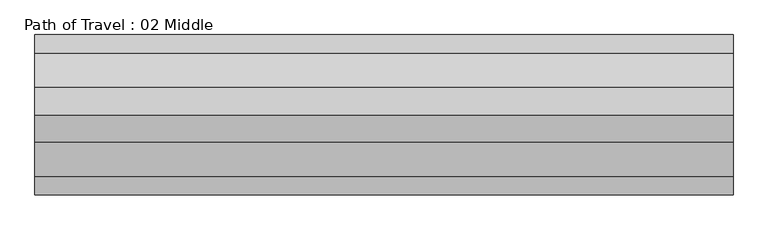
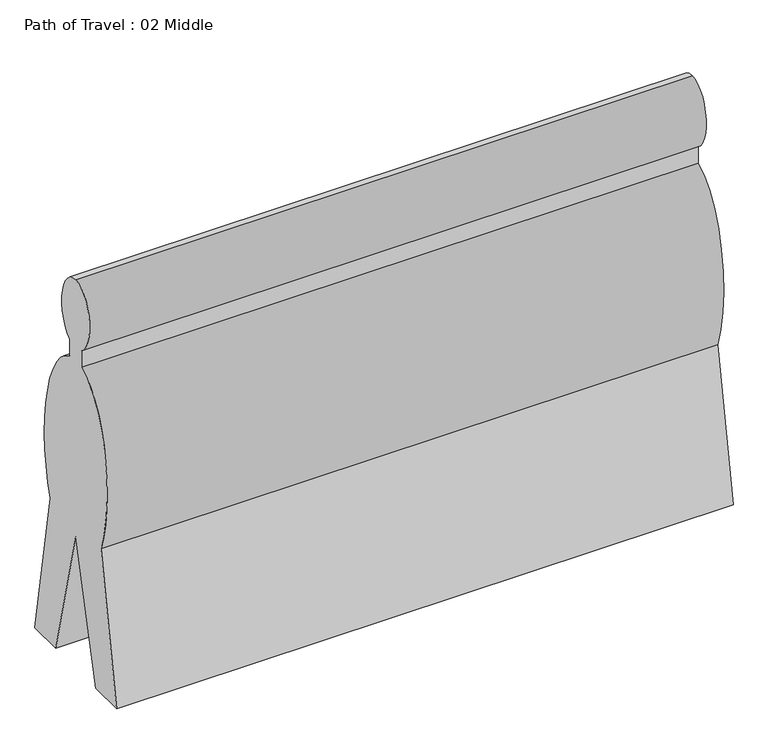
"""IFC4 building model written with IfcOpenShell, lengths in millimetres: proxy geometry, Path of Travel : 02 Middle."""

from ifc_helpers import new_model, si_unit, point, frame, origin, place, context, project, spatial, ellipse_curve, trimmed, source, transform, mapped, element, save
from ifc_brep_helpers import plane_surface, extruded_surface, advanced_brep


def path_of_travel_02_middle_fab60197(model_context):
    return source(origin(), model_context, "Body", "AdvancedBrep", [
        advanced_brep(
        [(227.5554837, 0.0, 1727.2), (227.5554837, 42.9018657, 1436.6534209), (227.5554837, 42.9018657, 1363.4763406), (227.5554837, 184.1186263, 643.4144547), (227.5554837, 297.5699544, 0.0), (227.5554837, 145.6574193, 0.0), (227.5554837, 0.0, 584.2), (227.5554837, -145.6574193, 0.0), (227.5554837, -297.5699544, 0.0), (227.5554837, -184.1186263, 643.4144547), (227.5554837, -42.9018657, 1363.4763406), (227.5554837, -42.9018657, 1436.6534209), (2818.3554837, 0.0, 1727.2), (2818.3554837, -42.9018657, 1436.6534209), (2818.3554837, -42.9018657, 1363.4763406), (2818.3554837, -184.1186263, 643.4144547), (2818.3554837, -297.5699544, 0.0), (2818.3554837, -145.6574193, 0.0), (2818.3554837, 0.0, 584.2), (2818.3554837, 145.6574193, 0.0), (2818.3554837, 297.5699544, 0.0), (2818.3554837, 184.1186263, 643.4144547), (2818.3554837, 42.9018657, 1363.4763406), (2818.3554837, 42.9018657, 1436.6534209)],
        [
            (0, 1, ellipse_curve(frame((227.5554837, 0.0, 1574.8), z_axis=(-1.0, 0.0, 0.0), x_axis=(0.0, 0.0, 1.0)), 152.4, 101.6)),
            (1, 2),
            (2, 3, ellipse_curve(frame((227.5554837, 0.0, 914.4), z_axis=(-1.0, 0.0, 0.0), x_axis=(0.0, 0.0, -1.0)), 457.2, 228.6)),
            (3, 4),
            (4, 5),
            (5, 6),
            (6, 7),
            (7, 8),
            (8, 9),
            (9, 10, ellipse_curve(frame((227.5554837, 0.0, 914.4), z_axis=(-1.0, 0.0, 0.0), x_axis=(0.0, 0.0, -1.0)), 457.2, 228.6)),
            (10, 11),
            (11, 0, ellipse_curve(frame((227.5554837, 0.0, 1574.8), z_axis=(-1.0, 0.0, 0.0), x_axis=(0.0, 0.0, 1.0)), 152.4, 101.6)),
            (12, 13, ellipse_curve(frame((2818.3554837, 0.0, 1574.8), z_axis=(1.0, 0.0, 0.0), x_axis=(0.0, 0.0, 1.0)), 152.4, 101.6)),
            (13, 14),
            (14, 15, ellipse_curve(frame((2818.3554837, 0.0, 914.4), z_axis=(1.0, 0.0, 0.0), x_axis=(0.0, 0.0, -1.0)), 457.2, 228.6)),
            (15, 16),
            (16, 17),
            (17, 18),
            (18, 19),
            (19, 20),
            (20, 21),
            (21, 22, ellipse_curve(frame((2818.3554837, 0.0, 914.4), z_axis=(1.0, 0.0, 0.0), x_axis=(0.0, 0.0, -1.0)), 457.2, 228.6)),
            (22, 23),
            (23, 12, ellipse_curve(frame((2818.3554837, 0.0, 1574.8), z_axis=(1.0, 0.0, 0.0), x_axis=(0.0, 0.0, 1.0)), 152.4, 101.6)),
            (0, 12),
            (23, 1),
            (22, 2),
            (21, 3),
            (20, 4),
            (19, 5),
            (18, 6),
            (17, 7),
            (16, 8),
            (15, 9),
            (14, 10),
            (13, 11),
        ],
        [
            plane_surface(frame((227.5554837, 0.0, 0.0), z_axis=(-1.0, 0.0, 0.0), x_axis=(0.0, 0.0, 1.0))),
            plane_surface(frame((2818.3554837, 0.0, 0.0), z_axis=(1.0, 0.0, 0.0), x_axis=(0.0, 0.0, 1.0))),
            extruded_surface(trimmed(ellipse_curve(frame((2818.3554837, 0.0, 1574.8), z_axis=(-1.0, 0.0, 0.0), x_axis=(0.0, 0.0, 1.0)), 152.4, 101.6), [point((2818.3554837, 0.0, 1727.2))], [point((2818.3554837, 42.9018657, 1436.6534209))], True, "CARTESIAN"), (-2590.8, 0.0, 0.0), 2590.8),
            plane_surface(frame((227.5554837, 42.9018657, 1436.6534209), z_axis=(0.0, 1.0, 0.0), x_axis=(1.0, 0.0, 0.0))),
            extruded_surface(trimmed(ellipse_curve(frame((2818.3554837, 0.0, 914.4), z_axis=(-1.0, 0.0, 0.0), x_axis=(0.0, 0.0, -1.0)), 457.2, 228.6), [point((2818.3554837, 42.9018657, 1363.4763406))], [point((2818.3554837, 184.1186263, 643.4144547))], True, "CARTESIAN"), (-2590.8, 0.0, 0.0), 2590.8),
            plane_surface(frame((227.5554837, 184.1186263, 643.4144547), z_axis=(0.0, 0.9848077530122078, 0.17364817766693205), x_axis=(1.0, 0.0, 0.0))),
            plane_surface(frame((227.5554837, 297.5699544, 0.0), z_axis=(0.0, 0.0, -1.0), x_axis=(1.0, 0.0, 0.0))),
            plane_surface(frame((227.5554837, 145.6574193, 0.0), z_axis=(0.0, -0.9702957262760199, -0.2419218955995739), x_axis=(1.0, 0.0, 0.0))),
            plane_surface(frame((227.5554837, 0.0, 584.2), z_axis=(0.0, 0.9702957262759961, -0.24192189559966923), x_axis=(1.0, 0.0, 0.0))),
            plane_surface(frame((227.5554837, -145.6574193, 0.0), z_axis=(0.0, 0.0, -1.0), x_axis=(1.0, 0.0, 0.0))),
            plane_surface(frame((227.5554837, -297.5699544, 0.0), z_axis=(0.0, -0.984807753012208, 0.17364817766693066), x_axis=(1.0, 0.0, 0.0))),
            extruded_surface(trimmed(ellipse_curve(frame((2818.3554837, 0.0, 914.4), z_axis=(-1.0, 0.0, 0.0), x_axis=(0.0, 0.0, -1.0)), 457.2, 228.6), [point((2818.3554837, -184.1186263, 643.4144547))], [point((2818.3554837, -42.9018657, 1363.4763406))], True, "CARTESIAN"), (-2590.8, 0.0, 0.0), 2590.8),
            plane_surface(frame((227.5554837, -42.9018657, 1363.4763406), z_axis=(0.0, -1.0, 0.0), x_axis=(1.0, 0.0, 0.0))),
            extruded_surface(trimmed(ellipse_curve(frame((2818.3554837, 0.0, 1574.8), z_axis=(-1.0, 0.0, 0.0), x_axis=(0.0, 0.0, 1.0)), 152.4, 101.6), [point((2818.3554837, -42.9018657, 1436.6534209))], [point((2818.3554837, 0.0, 1727.2))], True, "CARTESIAN"), (-2590.8, 0.0, 0.0), 2590.8),
        ],
        [
            (0, [[1, 2, 3, 4, 5, 6, 7, 8, 9, 10, 11, 12]]),
            (1, [[13, 14, 15, 16, 17, 18, 19, 20, 21, 22, 23, 24]]),
            (2, [[-1, 25, -24, 26]]),
            (3, [[-2, -26, -23, 27]]),
            (4, [[-3, -27, -22, 28]]),
            (5, [[-4, -28, -21, 29]]),
            (6, [[-5, -29, -20, 30]]),
            (7, [[-6, -30, -19, 31]]),
            (8, [[-7, -31, -18, 32]]),
            (9, [[-8, -32, -17, 33]]),
            (10, [[-9, -33, -16, 34]]),
            (11, [[-10, -34, -15, 35]]),
            (12, [[-11, -35, -14, 36]]),
            (13, [[-12, -36, -13, -25]]),
        ],
    ),
    ])


if __name__ == "__main__":
    model = new_model("IFC4")
    model_context = context("Model", 3, world=origin())
    ifc_project = project(units=[si_unit("LENGTHUNIT", "METRE", prefix="MILLI")], contexts=[model_context])
    site = spatial("IfcSite", under=ifc_project)
    building = spatial("IfcBuilding", under=site)
    placement = place(None, origin())
    path_of_travel_02_middle_shape = path_of_travel_02_middle_fab60197(model_context)
    element("IfcBuildingElementProxy", 1, Name="Path of Travel : 02 Middle", ObjectType="Path of Travel : 02 Middle", at=placement, inside=building, context=model_context, shape_type="MappedRepresentation", body=[
        mapped(path_of_travel_02_middle_shape, transform((0.0, 0.0, 0.0), x_axis=(1.0, 0.0, 0.0), y_axis=(0.0, 1.0, 0.0), z_axis=(0.0, 0.0, 1.0))),
    ])
    save(model, "model.ifc")

# Revit data of these elements
# Type "Path of Travel : 02 Middle"
#   Path of Egress [instance default] = 4' - 0"
#   built-in parameter 1001306 [instance default] = 4 (stored number, unit not read)
#   Dot at Start = no
#   Arrow in Middle = yes
#   Arrow at End = no
#   Egress Path = none
# Element 1 (IfcBuildingElementProxy, "Path of Travel : 02 Middle")
#   Path of Egress = 8' - 6"
#   built-in parameter 1001306 = 8.5 (stored number, unit not read)
#   Materials on its faces: "Egress Path Solid"
# Materials
#   "Egress Path Solid": class "Unassigned", colour RGB 255 128 64, transparency 0.75, Comments = "Rendering appearance not upgraded "
